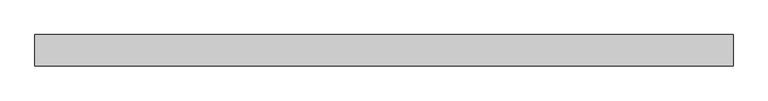
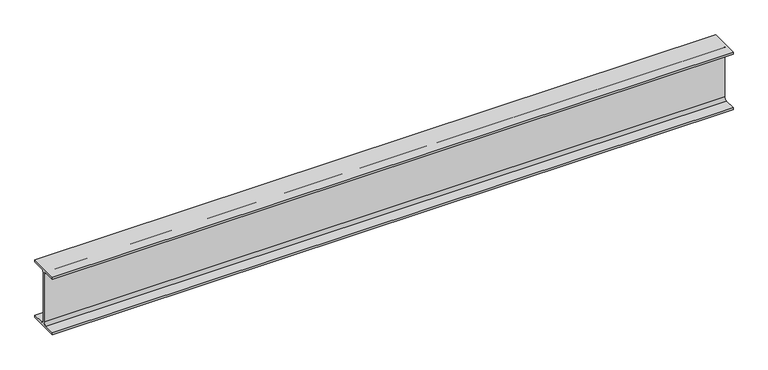
"""IFC4 building model written with IfcOpenShell, lengths in millimetres: beam geometry, 0912_Steel Framing_H-KSD3502 : H_SB_ASB_H-250x125x6x9."""

from ifc_helpers import new_model, si_unit, point, frame, frame_2d, origin, place, context, project, spatial, polyline, circle_curve, trimmed, segment, composite_curve, outline, extrude, source, transform, mapped, element, save


def beam_4887c4f3(model_context):
    return source(origin(), model_context, "Body", "SweptSolid", [
        extrude(outline(composite_curve([segment(polyline([(62.5, -116.0), (62.5, -125.0), (-62.5, -125.0), (-62.5, -116.0), (-15.0, -116.0)]), True, "CONTINUOUS"), segment(trimmed(circle_curve(frame_2d((-15.0, -104.0)), 12.0), [point((-15.0, -116.0))], [point((-3.0, -104.0))], True, "CARTESIAN"), True, "CONTINUOUS"), segment(polyline([(-3.0, -104.0), (-3.0, 104.0)]), True, "CONTINUOUS"), segment(trimmed(circle_curve(frame_2d((-15.0, 104.0)), 12.0), [point((-3.0, 104.0))], [point((-15.0, 116.0))], True, "CARTESIAN"), True, "CONTINUOUS"), segment(polyline([(-15.0, 116.0), (-62.5, 116.0), (-62.5, 125.0), (62.5, 125.0), (62.5, 116.0), (15.0, 116.0)]), True, "CONTINUOUS"), segment(trimmed(circle_curve(frame_2d((15.0, 104.0)), 12.0), [point((15.0, 116.0))], [point((3.0, 104.0))], True, "CARTESIAN"), True, "CONTINUOUS"), segment(polyline([(3.0, 104.0), (3.0, -104.0)]), True, "CONTINUOUS"), segment(trimmed(circle_curve(frame_2d((15.0, -104.0)), 12.0), [point((3.0, -104.0))], [point((15.0, -116.0))], True, "CARTESIAN"), True, "CONTINUOUS"), segment(polyline([(15.0, -116.0), (62.5, -116.0)]), True, "CONTINUOUS")], self_intersect=False)), frame((-1382.298157, 0.0, 0.0), z_axis=(1.0, 0.0, 0.0), x_axis=(0.0, 1.0, 0.0)), (0.0, 0.0, 1.0), 2794.5982),
    ])


if __name__ == "__main__":
    model = new_model("IFC4")
    model_context = context("Model", 3, world=origin())
    ifc_project = project(units=[si_unit("LENGTHUNIT", "METRE", prefix="MILLI")], contexts=[model_context])
    site = spatial("IfcSite", under=ifc_project)
    building = spatial("IfcBuilding", under=site)
    placement = place(None, origin())
    beam_shape = beam_4887c4f3(model_context)
    element("IfcBeam", 1, ObjectType="0912_Steel Framing_H-KSD3502 : H_SB_ASB_H-250x125x6x9", at=placement, inside=building, context=model_context, shape_type="MappedRepresentation", body=[
        mapped(beam_shape, transform((0.0, 0.0, 0.0), x_axis=(1.0, 0.0, 0.0), y_axis=(0.0, 1.0, 0.0), z_axis=(0.0, 0.0, 1.0))),
    ])
    save(model, "model.ifc")

# Revit data of these elements
# Type "0912_Steel Framing_H-KSD3502 : H_SB_ASB_H-250x125x6x9"
#   H_WM Code_1 = "S01AA003-00001 | Main Steel Structure Fabrication Work | Shelter/Building | Light Steel - Standard (30KG/M>Weight) | Material: (   )"
#   H_WM Code_2 = "S03AA029-00001 | Main Steel Structure Erection Work | Shelter/Building | Light Steel (30KG/M>Weight) | Material: (   )"
#   H_WM Code_3 = "S01AA010-00001 | Main Steel Structure Fabrication Work | Shelter/Building | Steel Painting/Coating | for Non-Fireproofed Steel Surface, Surface Preparation, Primer, Second & Final Coat | Material: (   )"
#   H_Q'ty Cal Type Tag = "SB-Q2"
#   Width = 12.5 cm
#   Web Thickness = 0.6 cm
#   Web Fillet = 1.2 cm
#   Warping Constant = 42539.8 cm⁶
#   W = 0
#   Torsional Moment of Inertia = 7.8102 cm⁴
#   Section Area = 37.66 cm²
#   Plastic Modulus weak axis = 73.1 cm³
#   Plastic Modulus strong axis = 366.0 cm³
#   Perimeter = 0.97 m²/m
#   Nominal Weight = 29.60 kgf/m
#   Moment of Inertia weak axis = 294.00 cm⁴
#   Moment of Inertia strong axis = 4050.00 cm⁴
#   Height = 25.0 cm
#   Flange Thickness = 0.9 cm
#   Elastic Modulus weak axis = 47.0 cm³
#   Elastic Modulus strong axis = 324.0 cm³
#   Centroid Vertical = 12.5 cm
#   Centroid Horizontal = 6.25 cm
#   Ix = 40500000
#   Length [instance default] = 1.5240 m
#   Zx = 366000
#   b = 0.1250 m
#   h = 0.2500 m
#   r = 0.0120 m
#   s = 0.0060 m
#   t = 0.0090 m
#   A = 0.003766 m²
#   Structural Material [instance default] = Steel, 45-345
#   Assembly Code = ""
# Element 1 (IfcBeam, "0912_Steel Framing_H-KSD3502 : H_SB_ASB_H-250x125x6x9")
#   Structural Material = none
# Materials
#   "Steel, 45-345": class "Metal", colour RGB 189 187 185, transparency 0, Description = "Steel 345 MPa", Cost = 0
